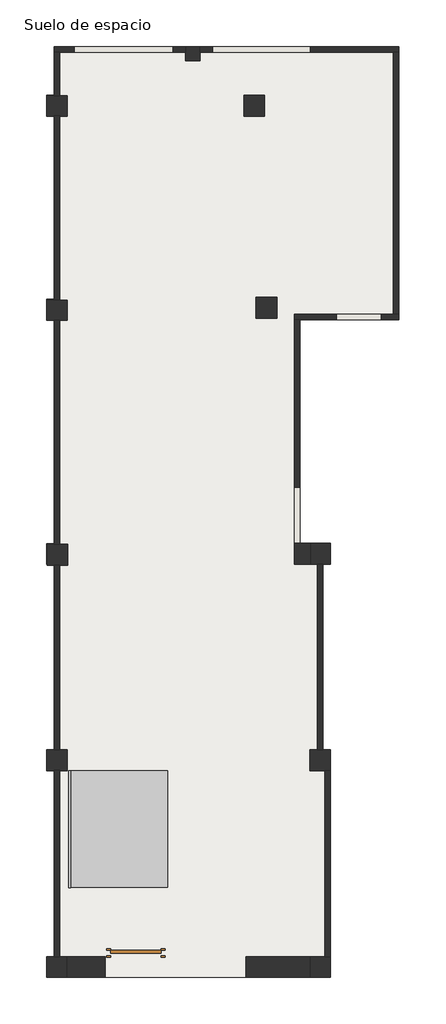
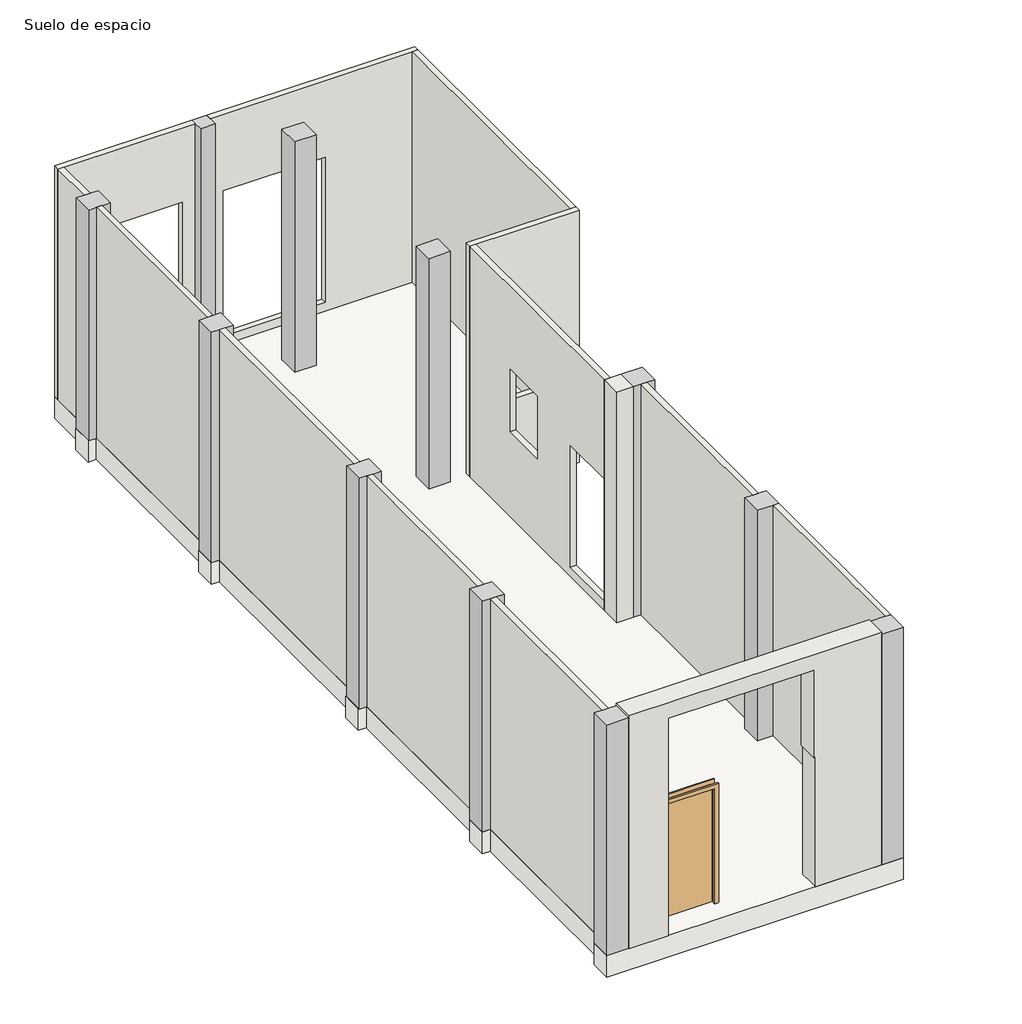
# One storey: 14 walls, 11 columns, 1 door, 1 railing, 1 ramp, 1 slab.
# Revit data of these elements (continued)
# Element 15 (IfcSlab, "Generic Floor - 400mm")
#   Height Offset From Level = 0.0 cm
#   Phase Created = New Construction
#   Materials on its faces: "Default Roof"
# Elements 16, 17, 18, 19, 20, 21, 22, 23, 24, 25, 26, 27 (IfcWall, "Generic - 100mm Masonry")
#   Top Offset = 0.0 cm
#   Base Offset = 0.0 cm
#   wall height = 426.0 cm
#   Phase Created = Existing
#   Base Constraint = Suelo de espacio
#   Top Constraint = Techo de espacio
#   Materials on its faces: "Concrete, Cast-in-Place gray"
# Element 28 (IfcWall, "Generic - 380mm Masonry")
#   Top Offset = 0.0 cm
#   Base Offset = 0.0 cm
#   wall height = 426.0 cm
#   Phase Created = Existing
#   Base Constraint = Suelo de espacio
#   Top Constraint = Techo de espacio
#   Materials on its faces: "Concrete, Cast-in-Place gray"
# Element 29 (IfcWall, "Generic - 380mm Masonry")
#   Top Offset = 0.0 cm
#   Base Offset = 0.0 cm
#   Unconnected Height = 430.0 cm
#   wall height = 430.0 cm
#   Phase Created = Existing
#   Base Constraint = Suelo de espacio
#   Materials on its faces: "Concrete, Cast-in-Place gray"
# Materials
#   "Door - Panel": class "Wood", colour RGB 114 82 51, transparency 0
#   "Door - Frame": class "Miscellaneous", colour RGB 153 76 43, transparency 0
#   "Concrete, Cast-in-Place gray": class "Concrete", colour RGB 115 116 108, transparency 0, Description = "Cast-in-place concrete", Cost = 0
#   "Default Roof": class "Miscellaneous", colour RGB 80 80 80, transparency 0
